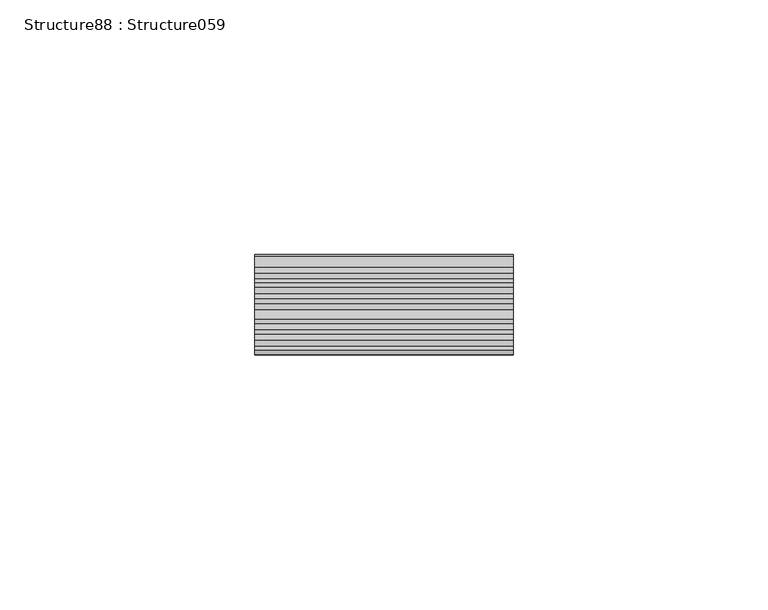
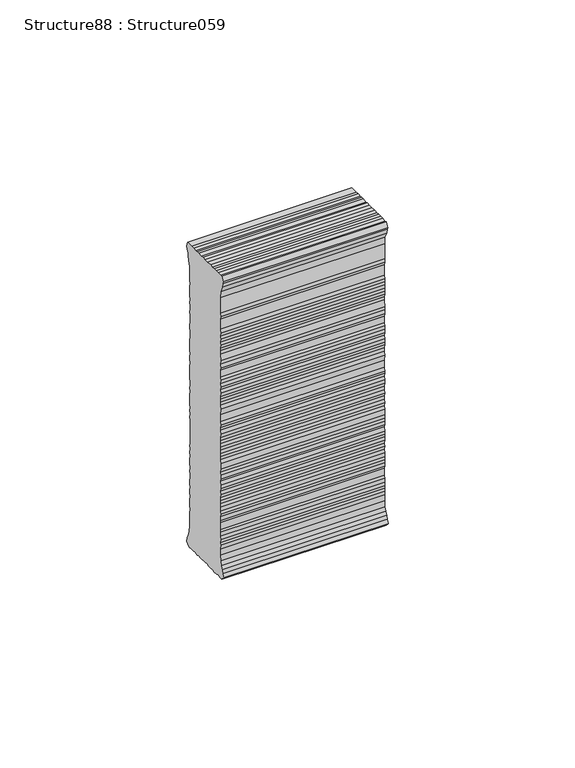
"""IFC4 building model written with IfcOpenShell, lengths in millimetres: proxy geometry, Structure88 : Structure059."""

from ifc_helpers import new_model, si_unit, frame, origin, place, context, project, spatial, polyline, outline, extrude, source, transform, mapped, element, save


def structure88_structure059_237fe73c(model_context):
    return source(origin(), model_context, "Body", "SweptSolid", [
        extrude(outline(polyline([(1.8231554, 0.0), (3.146451, 0.2948314), (4.223301, 0.7409331), (5.4047307, 0.9167105), (6.4772964, 1.3627598), (7.4528114, 0.3820762), (7.3884057, -0.5247488), (7.0434645, -1.6749028), (7.2501163, -2.4718494), (7.1673846, -3.6367026), (6.9649918, -4.6632138), (7.0294228, -5.5791892), (6.8268536, -6.6081849), (6.629201, -7.5076866), (6.6888666, -8.5510265), (6.5229999, -10.8864115), (6.316449, -11.9112006), (6.523126, -12.7077923), (6.1783108, -13.8561716), (6.2561259, -14.6439679), (6.1641178, -15.9394323), (6.2193731, -16.9845992), (6.0352812, -17.7534372), (5.0780922, -18.3378809), (3.7953527, -18.1169333), (2.7962655, -17.5233917), (1.913164, -17.0697144), (1.0339666, -16.6163146), (-1.0179911, -16.2116049), (-2.0536528, -16.1380488), (-3.1025726, -16.1908972), (-5.1724761, -16.0438859), (-6.3290923, -15.7045498), (-7.5013464, -15.7511357), (-8.4171706, -15.813437), (-9.3239956, -15.7490313), (-10.601995, -15.4010742), (-11.6561864, -15.5833915), (-12.6957522, -15.5095581), (-13.5787236, -15.1896571), (-14.500758, -15.2540145), (-15.6638365, -15.1714088), (-16.6906774, -14.968636), (-17.7302432, -14.8948026), (-18.7736607, -14.9505389), (-19.9293382, -14.7386156), (-20.9874337, -14.9206557), (-21.8942587, -14.85625), (-22.7920846, -14.6651373), (-23.8171509, -14.4624904), (-24.862343, -14.5181007), (-26.0258289, -14.3056229), (-26.9379254, -14.370686), (-28.097507, -14.1584855), (-35.4862676, -13.6337114), (-36.2730768, -13.7076729), (-37.56185, -13.4862968), (-38.6049127, -13.5420583), (-39.3758549, -13.3574602), (-40.5481091, -13.4040461), (-41.4639333, -13.4663475), (-42.4948548, -13.2657818), (-43.6669324, -13.3098832), (-44.8136108, -12.9712529), (-45.7335156, -13.0357615), (-46.8874186, -12.8239643), (-47.9269843, -12.7501309), (-48.9811756, -12.9324482), (-50.9279214, -12.7941839), (-51.822198, -12.6033233), (-53.1180172, -12.51129), (-54.0160215, -12.3176675), (-55.1939545, -12.3638501), (-56.2281963, -12.2903948), (-57.1258459, -12.0967975), (-58.0414915, -12.1616087), (-60.3797159, -11.9955403), (-61.418343, -12.0491198), (-62.4404439, -11.7193373), (-64.2597726, -11.5901226), (-65.4323817, -11.6366834), (-66.3425272, -11.699388), (-67.4987884, -11.3600771), (-69.568692, -11.2130658), (-70.4940467, -11.4045335), (-71.7716912, -11.0566015), (-72.8073527, -10.9830454), (-73.5945168, -11.0569817), (-74.7487746, -10.8451593), (-75.7996455, -10.9003662), (-76.7154697, -10.9626676), (-78.918114, -10.8062286), (-79.8067643, -10.4859243), (-80.9846972, -10.5321069), (-85.2575999, -10.2286313), (-87.1143914, -10.616842), (-88.4338333, -10.9126605), (-89.3541939, -10.9785635), (-90.2847425, -11.3034293), (-91.3371067, -11.4901569), (-92.6113068, -11.0083459), (-92.4548678, -8.8057016), (-92.5012015, -7.6298982), (-92.2982775, -6.6009278), (-92.3722137, -5.8137638), (-92.3077828, -4.9065838), (-91.9594959, -3.6289645), (-92.1513185, -2.7035846), (-91.948571, -1.6770986), (-91.7387772, -0.5212698), (-91.8660681, 1.3127098), (-91.5453837, 2.2016897), (-91.7187795, 3.3865174), (-91.5250311, 4.2862964), (-91.5714908, 5.4603252), (-91.2323544, 6.6091078), (-91.4333526, 7.4052962), (-89.9470277, 8.0820021), (-89.2007223, 7.6359004), (-87.9140786, 7.4146756), (-85.9177564, 6.2316476), (-83.8509695, 5.9553712), (-78.9274953, 5.6056898), (-77.7492326, 5.6514922), (-76.8612147, 5.3273091), (-73.4894581, 5.0878358), (-72.4346346, 5.274032), (-71.4102529, 5.0717906), (-70.4939226, 5.1361963), (-69.3343157, 4.9243507), (-68.4179854, 4.9887564), (-67.3911193, 4.7863385), (-66.4932409, 4.5909415), (-65.4536751, 4.5171082), (-63.3653195, 4.6298995), (-62.2057127, 4.4180539), (-61.0331289, 4.4642597), (-60.139432, 4.1396732), (-57.9421116, 3.9836123), (-57.1438965, 4.1880336), (-55.8572276, 3.9671637), (-54.8117057, 4.0223938), (-53.9197836, 3.6979333), (-52.8653149, 3.8841547), (-51.7113868, 3.6727125), (-50.8045618, 3.6083068), (-49.777492, 3.4037342), (-48.7379263, 3.3299008), (-47.5507169, 3.5066945), (-45.755164, 3.1180552), (-43.4233281, 2.9524406), (-42.3709891, 3.1388132), (-41.6000215, 2.9545701), (-40.5694025, 2.7497454), (-39.5170634, 2.9361181), (-38.2342987, 2.7155254), (-37.2036797, 2.5107007), (-36.1676632, 2.4371194), (-35.122345, 2.4945043), (-34.0920809, 2.2897048), (-33.0578389, 2.2162495), (-32.0089715, 2.2733822), (-30.9822567, 2.0688348), (-29.927788, 2.2550562), (-28.1137831, 2.1262196), (-26.9559508, 1.9145001), (-26.0399754, 1.978931), (-24.8751223, 1.8961993), (-23.9828451, 1.5717137), (-22.8013146, 1.7489107), (-21.765298, 1.6753294), (-20.8615898, 1.4816586), (-19.8185523, 1.5370651), (-18.6682471, 1.1942535), (-17.7517654, 1.2607887), (-16.7250506, 1.0562413), (-15.6818619, 1.1137773), (-14.3860427, 1.021744), (-13.4697123, 1.0861497), (-12.4371674, 0.8833285), (-11.2740889, 0.8007228), (-10.5057571, 0.6145266), (-8.1735663, 0.4488868), (-7.3845017, 0.5244716), (-6.0886824, 0.4324382), (-5.0435154, 0.4876935), (-4.0127452, 0.2849983), (-3.2295105, 0.3588569), (-1.9428416, 0.137987), (0.0, 0.0), (1.8231554, 0.0)])), frame((-56111.1523075, 292059.2626311, -368.1935385), z_axis=(-0.9999998917542984, 0.0004652863545059615, 0.0), x_axis=(-3.296313100390944e-05, -0.07084481872518561, -0.9974873485780297)), (0.0, 0.0, 1.0), 50.8),
    ])


if __name__ == "__main__":
    model = new_model("IFC4")
    model_context = context("Model", 3, world=origin())
    ifc_project = project(units=[si_unit("LENGTHUNIT", "METRE", prefix="MILLI")], contexts=[model_context])
    site = spatial("IfcSite", under=ifc_project)
    building = spatial("IfcBuilding", under=site)
    placement = place(None, origin())
    structure88_structure059_shape = structure88_structure059_237fe73c(model_context)
    element("IfcBuildingElementProxy", 1, Name="Structure88 : Structure059", ObjectType="Structure88 : Structure059", at=placement, inside=building, context=model_context, shape_type="MappedRepresentation", body=[
        mapped(structure88_structure059_shape, transform((0.0, 0.0, 0.0), x_axis=(1.0, 0.0, 0.0), y_axis=(0.0, 1.0, 0.0), z_axis=(0.0, 0.0, 1.0))),
    ])
    save(model, "model.ifc")

# Revit data of these elements
# Type "Structure88 : Structure059"
#   NameOverride = "Structure059"
# Element 1 (IfcBuildingElementProxy, "Structure88 : Structure059")
#   Materials on its faces: "BRUSHED ALUMINUM LETTERING"
# Materials
#   "BRUSHED ALUMINUM LETTERING": class "Unassigned", colour RGB 169 181 186, transparency 0, Cost = 0
